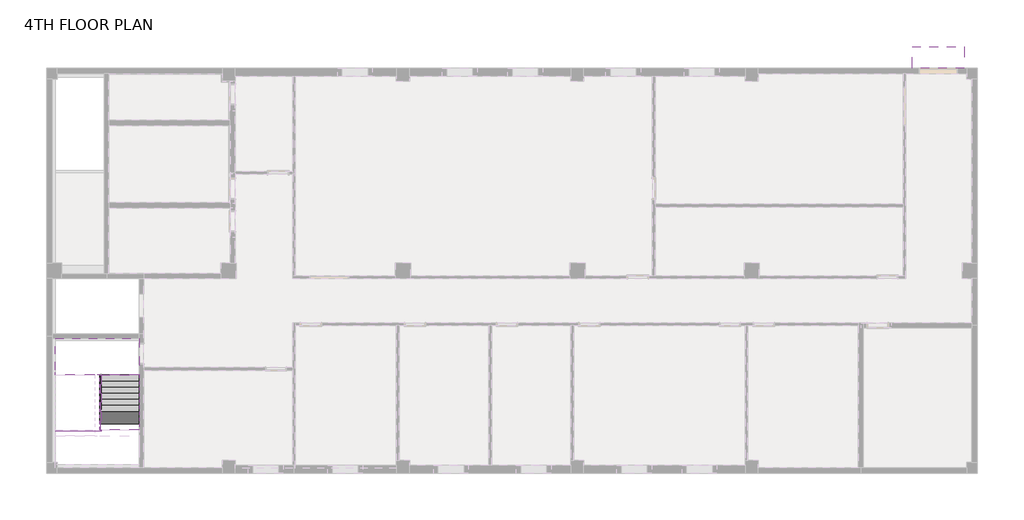
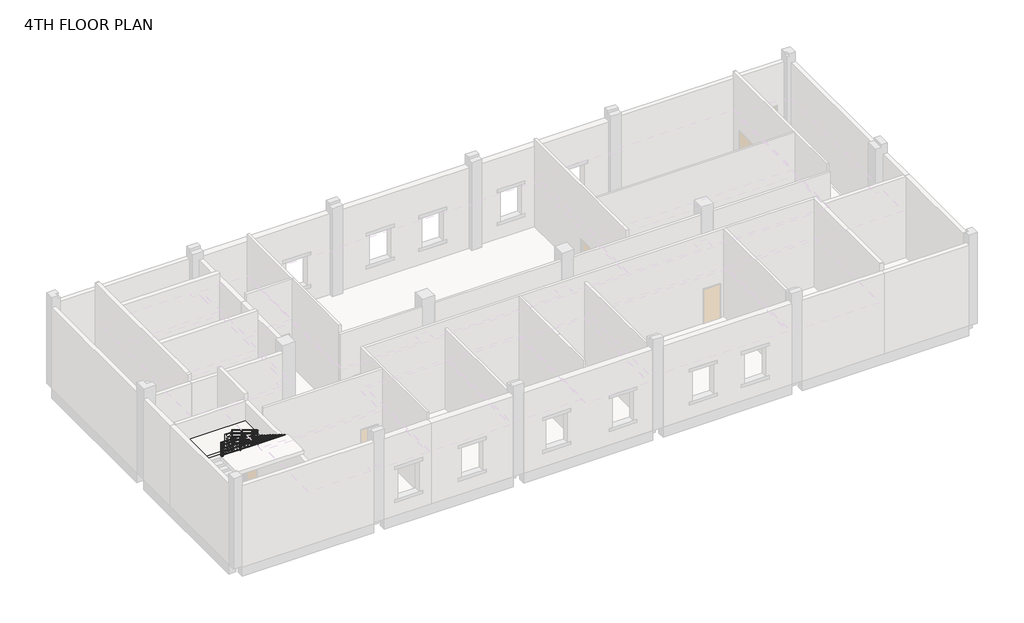
# One storey, part 6 of 6: 2 stair flights, 1 proxy, 1 railing, 1 slab.
"""IFC4 building model written with IfcOpenShell, lengths in millimetres."""

import ifcopenshell
import ifcopenshell.guid

model = None  # the IFC model being written
_history = None  # IfcOwnerHistory: only IFC2X3 demands one
_inside = {}  # id of a spatial element -> (the spatial element, [elements in it])
_under = {}  # id of a project, library or spatial element -> (it, [spatial elements below it])
_declared = {}  # id of a project -> (the project, [libraries it declares])
_typed = {}  # id of a type object -> (the type object, [elements of that type])
_made_of = {}  # id of a material, layer set ... -> (it, [elements and type objects made of it])


def new_model(schema):
    """Start an empty IFC model of exactly this schema.

    Asked for "IFC4X3", IfcOpenShell would pick the latest addendum, in which some entities
    have other attributes; the version numbers below select the first issue.
    IFC2X3 requires an IfcOwnerHistory on every rooted entity: one is made here for all.
    """
    global model, _history
    if schema == "IFC4X3":
        model = ifcopenshell.file(schema_version=(4, 3, 0, 0))
    else:
        model = ifcopenshell.file(schema=schema)
    _inside.clear()
    _under.clear()
    _declared.clear()
    _typed.clear()
    _made_of.clear()
    _history = None
    if model.schema == "IFC2X3":
        org = make("IfcOrganization", Name="unknown")
        user = make(
            "IfcPersonAndOrganization",
            ThePerson=make("IfcPerson", FamilyName="unknown"),
            TheOrganization=org,
        )
        app = make(
            "IfcApplication",
            ApplicationDeveloper=org,
            Version="unknown",
            ApplicationFullName="unknown",
            ApplicationIdentifier="unknown",
        )
        _history = make(
            "IfcOwnerHistory",
            OwningUser=user,
            OwningApplication=app,
            ChangeAction="ADDED",
            CreationDate=0,
        )
    return model


def make(cls, **values):
    """One entity of the class cls with the attributes given. An attribute that is None is left unset."""
    return model.create_entity(
        cls, **{name: value for name, value in values.items() if value is not None}
    )


def rooted(cls, **values):
    """An entity with a GlobalId (a new one), such as an element, a storey or a relation."""
    return make(cls, GlobalId=ifcopenshell.guid.new(), OwnerHistory=_history, **values)


def si_unit(unit_type, name, prefix=None):
    """IfcSIUnit, for example si_unit("LENGTHUNIT", "METRE", prefix="MILLI")."""
    return make("IfcSIUnit", UnitType=unit_type, Prefix=prefix, Name=name)


def assignment(units):
    """IfcUnitAssignment: the units of a project."""
    return None if units is None else make("IfcUnitAssignment", Units=units)


def point(xyz):
    """IfcCartesianPoint."""
    return None if xyz is None else make("IfcCartesianPoint", Coordinates=xyz)


def direction(xyz):
    """IfcDirection."""
    return None if xyz is None else make("IfcDirection", DirectionRatios=xyz)


def frame(location, z_axis=None, x_axis=None):
    """IfcAxis2Placement3D, a coordinate frame: its origin and axes. An axis left out is left unset."""
    return make(
        "IfcAxis2Placement3D",
        Location=point(location),
        Axis=direction(z_axis),
        RefDirection=direction(x_axis),
    )


def origin():
    """The frame at (0, 0, 0) with its axes left unset."""
    return frame((0.0, 0.0, 0.0))


def place(relative_to, where):
    """IfcLocalPlacement: puts the frame where relative to a parent placement (None: the world)."""
    return make(
        "IfcLocalPlacement", PlacementRelTo=relative_to, RelativePlacement=where
    )


def context(
    kind, dimensions, precision=None, world=None, true_north=None, identifier=None
):
    """IfcGeometricRepresentationContext, for example the 3D "Model" context."""
    return make(
        "IfcGeometricRepresentationContext",
        ContextIdentifier=identifier,
        ContextType=kind,
        CoordinateSpaceDimension=dimensions,
        Precision=precision,
        WorldCoordinateSystem=world,
        TrueNorth=true_north,
    )


def project(units=None, contexts=None):
    """IfcProject with its units and contexts."""
    return rooted(
        "IfcProject",
        Name="project",
        RepresentationContexts=contexts,
        UnitsInContext=assignment(units),
    )


def spatial(cls, under=None, at=None, **own):
    """A site, building, storey or space (cls), placed at a placement, below another one or the project."""
    s = rooted(cls, ObjectPlacement=at, **own)
    if under is not None:
        _under.setdefault(under.id(), (under, []))[1].append(s)
    return s


def polyline(points):
    """IfcPolyline through the points."""
    return make("IfcPolyline", Points=[point(p) for p in points])


def circle_curve(where, radius):
    """IfcCircle in the frame where."""
    return make("IfcCircle", Position=where, Radius=radius)


def ellipse_curve(where, semi_axis1, semi_axis2):
    """IfcEllipse in the frame where."""
    return make(
        "IfcEllipse", Position=where, SemiAxis1=semi_axis1, SemiAxis2=semi_axis2
    )


def outline(outer, holes=None, kind="AREA"):
    """IfcArbitraryClosedProfileDef: a profile drawn as a closed curve; with holes, ...WithVoids."""
    if holes is None:
        return make("IfcArbitraryClosedProfileDef", ProfileType=kind, OuterCurve=outer)
    return make(
        "IfcArbitraryProfileDefWithVoids",
        ProfileType=kind,
        OuterCurve=outer,
        InnerCurves=holes,
    )


def extrude(swept, where, along, depth):
    """IfcExtrudedAreaSolid: the profile swept, set in the frame where, extruded along a direction by depth."""
    return make(
        "IfcExtrudedAreaSolid",
        SweptArea=swept,
        Position=where,
        ExtrudedDirection=direction(along),
        Depth=depth,
    )


def faces_of(points, faces, orient=None, outer=None):
    """IfcFace entities. A face is a list of loops; a loop is a list of indices into points, from 0.

    orient and outer hold one flag for each loop. By default every Orientation is true, the
    first loop of a face is its IfcFaceOuterBound and the others are IfcFaceBound.
    """
    made = []
    for i, loops in enumerate(faces):
        bounds = []
        for j, loop in enumerate(loops):
            is_outer = j == 0 if outer is None else outer[i][j]
            bounds.append(
                make(
                    "IfcFaceOuterBound" if is_outer else "IfcFaceBound",
                    Bound=make("IfcPolyLoop", Polygon=[points[k] for k in loop]),
                    Orientation=True if orient is None else orient[i][j],
                )
            )
        made.append(make("IfcFace", Bounds=bounds))
    return made


def faceted_brep(points, faces, orient=None, outer=None, voids=None):
    """IfcFacetedBrep: a solid bounded by flat faces; with voids (closed shells), ...WithVoids."""
    shared = [point(p) for p in points]
    hull = make("IfcClosedShell", CfsFaces=faces_of(shared, faces, orient, outer))
    if voids is None:
        return make("IfcFacetedBrep", Outer=hull)
    return make(
        "IfcFacetedBrepWithVoids",
        Outer=hull,
        Voids=[
            make(cls, CfsFaces=faces_of(shared, fs, o, b)) for cls, fs, o, b in voids
        ],
    )


def shape(context_of_items, identifier, shape_type, items):
    """IfcShapeRepresentation: the items that make up one representation, for example the "Body"."""
    return make(
        "IfcShapeRepresentation",
        ContextOfItems=context_of_items,
        RepresentationIdentifier=identifier,
        RepresentationType=shape_type,
        Items=items,
    )


def source(mapping_origin, context_of_items, identifier, shape_type, items):
    """IfcRepresentationMap: a shape defined once, which mapped items show again and again."""
    return make(
        "IfcRepresentationMap",
        MappingOrigin=mapping_origin,
        MappedRepresentation=shape(context_of_items, identifier, shape_type, items),
    )


def transform(
    local_origin,
    x_axis=None,
    y_axis=None,
    z_axis=None,
    scale=None,
    scale2=None,
    scale3=None,
    uniform=True,
):
    """IfcCartesianTransformationOperator3D, or its non-uniform kind. x_axis, y_axis, z_axis: its Axis1, 2, 3."""
    if uniform:
        return make(
            "IfcCartesianTransformationOperator3D",
            Axis1=direction(x_axis),
            Axis2=direction(y_axis),
            LocalOrigin=point(local_origin),
            Scale=scale,
            Axis3=direction(z_axis),
        )
    return make(
        "IfcCartesianTransformationOperator3DnonUniform",
        Axis1=direction(x_axis),
        Axis2=direction(y_axis),
        LocalOrigin=point(local_origin),
        Scale=scale,
        Axis3=direction(z_axis),
        Scale2=scale2,
        Scale3=scale3,
    )


def mapped(mapping_source, mapping_target):
    """IfcMappedItem: shows the shape of a source again, moved by a transform."""
    return make(
        "IfcMappedItem", MappingSource=mapping_source, MappingTarget=mapping_target
    )


def made_of(thing, what):
    """Note that an element or type object is made of a material, layer set ...; save() writes the relation."""
    if what is not None:
        _made_of.setdefault(what.id(), (what, []))[1].append(thing)
    return thing


def element(
    cls,
    number,
    at=None,
    inside=None,
    cuts=None,
    type_object=None,
    material=None,
    context=None,
    identifier="Body",
    shape_type=None,
    held_by="IfcProductDefinitionShape",
    body=None,
    shapes=None,
    **own,
):
    """One element of the class cls, such as IfcWall. Its Tag is "e" and its number.

    at: its placement. inside: the storey or other place that contains it. cuts: it is an
    opening in that element (IfcRelVoidsElement). A single representation is given by context,
    identifier, shape_type and body (its items); several are given by shapes. held_by: the class
    of the entity that holds the representations. save() writes the other relations.
    """
    e = rooted(cls, Tag="e%d" % number, ObjectPlacement=at, **own)
    if body is not None:
        shapes = [shape(context, identifier, shape_type, body)]
    if shapes is not None:
        e.Representation = make(held_by, Representations=shapes)
    if inside is not None:
        _inside.setdefault(inside.id(), (inside, []))[1].append(e)
    if cuts is not None:
        rooted(
            "IfcRelVoidsElement", RelatingBuildingElement=cuts, RelatedOpeningElement=e
        )
    if type_object is not None:
        _typed.setdefault(type_object.id(), (type_object, []))[1].append(e)
    return made_of(e, material)


def aggregate(whole, parts):
    """IfcRelAggregates: a whole, such as a stair, and the parts it consists of."""
    return rooted("IfcRelAggregates", RelatingObject=whole, RelatedObjects=parts)


def save(model, path):
    """Write the relations noted so far, then the file.

    IfcRelAggregates (storeys below a building ...), IfcRelContainedInSpatialStructure (elements
    in a storey), IfcRelDefinesByType, IfcRelAssociatesMaterial and IfcRelDeclares: one each for
    every whole, place, type object, material and project.
    """
    for whole, parts in _under.values():
        aggregate(whole, parts)
    for where, things in _inside.values():
        rooted(
            "IfcRelContainedInSpatialStructure",
            RelatedElements=things,
            RelatingStructure=where,
        )
    for kind, things in _typed.values():
        rooted("IfcRelDefinesByType", RelatedObjects=things, RelatingType=kind)
    for what, things in _made_of.values():
        rooted("IfcRelAssociatesMaterial", RelatedObjects=things, RelatingMaterial=what)
    for by, libraries in _declared.values():
        rooted("IfcRelDeclares", RelatingContext=by, RelatedDefinitions=libraries)
    model.write(path)


def plane_surface(at):
    """IfcPlane: the flat surface through the origin of the frame at, square to its z axis."""
    return make("IfcPlane", Position=at)


def cylinder_surface(at, radius):
    """IfcCylindricalSurface: all points at the distance radius from the z axis of the frame at."""
    return make("IfcCylindricalSurface", Position=at, Radius=radius)


def advanced_brep(points, edges, surfaces, faces):
    """IfcAdvancedBrep: a solid bounded by faces that lie on surfaces and meet in shared edges.

    An edge is (start, end): straight between two places in points (the first is 0);
    or (start, end, curve); or (start, end, curve, False) where it runs against its curve.
    A face is (place in surfaces, loops), or (place, loops, False) where it looks against
    its surface's normal. A loop lists edges by number (the first is 1), with a minus sign
    where the edge is run from its end to its start. The first loop is the outer one.
    """
    corners = [point(p) for p in points]
    vertices = [make("IfcVertexPoint", VertexGeometry=c) for c in corners]
    made = []
    for start, end, *more in edges:
        made.append(
            make(
                "IfcEdgeCurve",
                EdgeStart=vertices[start],
                EdgeEnd=vertices[end],
                EdgeGeometry=more[0] if more else make("IfcPolyline", Points=[corners[start], corners[end]]),
                SameSense=more[1] if len(more) > 1 else True,
            )
        )
    hull = []
    for where, loops, *sense in faces:
        bounds = []
        for j, loop in enumerate(loops):
            ring = [make("IfcOrientedEdge", EdgeElement=made[abs(k) - 1], Orientation=k > 0) for k in loop]
            bounds.append(
                make(
                    "IfcFaceOuterBound" if j == 0 else "IfcFaceBound",
                    Bound=make("IfcEdgeLoop", EdgeList=ring),
                    Orientation=True,
                )
            )
        hull.append(make("IfcAdvancedFace", Bounds=bounds, FaceSurface=surfaces[where], SameSense=sense[0] if sense else True))
    return make("IfcAdvancedBrep", Outer=make("IfcClosedShell", CfsFaces=hull))


def canopy_no_lintel2_canopy_no_lintel_c6626c79(model_context):
    return source(origin(), model_context, "Body", "SweptSolid", [
        extrude(outline(polyline([(-30.0, 1000.0), (0.0, 0.0), (-150.0, 0.0), (-150.0, 1000.0), (-30.0, 1000.0)])), frame((0.0, 0.0, 0.0), z_axis=(1.0, 0.0, 0.0), x_axis=(0.0, 1.0, 0.0)), (0.0, 0.0, 1.0), 2400.0),
    ])


model = new_model("IFC4")

# Units and contexts
model_context = context("Model", 3, world=origin())
ifc_project = project(units=[si_unit("LENGTHUNIT", "METRE", prefix="MILLI")], contexts=[model_context])

# Site, building, storey
site = spatial("IfcSite", under=ifc_project)
building = spatial("IfcBuilding", under=site)
storey = spatial("IfcBuildingStorey", under=building, Name="4TH FLOOR PLAN", Elevation=16100.005241)

# Proxy
placement = place(None, origin())
canopy_no_lintel2_canopy_no_lintel_shape = canopy_no_lintel2_canopy_no_lintel_c6626c79(model_context)
element("IfcBuildingElementProxy", 1, Name="Canopy_no_ Lintel2 : Canopy No Lintel", ObjectType="Canopy_no_ Lintel2 : Canopy No Lintel", at=placement, inside=storey, context=model_context, shape_type="MappedRepresentation", body=[
    mapped(canopy_no_lintel2_canopy_no_lintel_shape, transform((41750.0, 39300.5208589, 18900.005241), x_axis=(-1.0, 0.0, 0.0), y_axis=(0.0, 0.0, 1.0), z_axis=(0.0, 1.0, 0.0))),
])

# Railing
element("IfcRailing", 2, ObjectType="900mm 배관", at=placement, inside=storey, context=model_context, shape_type="SolidModel", body=[
    advanced_brep(
    [(2135.0, 25213.5208589, 20935.5296813), (2165.0, 25213.5208589, 20935.5296813), (2135.0, 22689.2843108, 22485.005241), (2165.0, 22689.2843108, 22485.005241), (2135.0, 22658.5208589, 22485.005241), (2165.0, 22628.5208589, 22485.005241), (50.0, 22658.5208589, 22485.005241), (50.0, 22628.5208589, 22485.005241)],
    [
        (0, 1, ellipse_curve(frame((2150.0, 25213.5208589, 20935.5296813), z_axis=(0.0, 1.0, 0.0), x_axis=(0.0, 0.0, -1.0)), 17.6005597, 15.0)),
        (1, 0, ellipse_curve(frame((2150.0, 25213.5208589, 20935.5296813), z_axis=(0.0, 1.0, 0.0), x_axis=(0.0, 0.0, -1.0)), 17.6005597, 15.0)),
        (0, 2),
        (2, 3, ellipse_curve(frame((2150.0, 22689.2843108, 22485.005241), z_axis=(0.0, 0.9623527489128064, -0.2718035810285896), x_axis=(0.0, -0.27180358102858976, -0.9623527489128063)), 15.5868002, 15.0)),
        (3, 1),
        (3, 2, ellipse_curve(frame((2150.0, 22689.2843108, 22485.005241), z_axis=(0.0, 0.9623527489128064, -0.2718035810285896), x_axis=(0.0, -0.27180358102858976, -0.9623527489128063)), 15.5868002, 15.0)),
        (2, 4),
        (4, 5, ellipse_curve(frame((2150.0, 22643.5208589, 22485.005241), z_axis=(0.7071067811865475, 0.7071067811865475, 0.0), x_axis=(-0.7071067811865474, 0.7071067811865476, 0.0)), 21.2132034, 15.0)),
        (5, 3),
        (5, 4, ellipse_curve(frame((2150.0, 22643.5208589, 22485.005241), z_axis=(0.7071067811865475, 0.7071067811865475, 0.0), x_axis=(-0.7071067811865474, 0.7071067811865476, 0.0)), 21.2132034, 15.0)),
        (6, 7, circle_curve(frame((50.0, 22643.5208589, 22485.005241), z_axis=(-1.0, 0.0, 0.0), x_axis=(0.0, -1.0, 0.0)), 15.0)),
        (7, 6, circle_curve(frame((50.0, 22643.5208589, 22485.005241), z_axis=(-1.0, 0.0, 0.0), x_axis=(0.0, -1.0, 0.0)), 15.0)),
        (4, 6),
        (7, 5),
    ],
    [
        plane_surface(frame((2150.0, 25213.5208589, 20953.130241), z_axis=(0.0, 1.0, 0.0), x_axis=(0.0, 0.0, -1.0))),
        cylinder_surface(frame((2150.0, 25205.6737312, 20940.3465566), z_axis=(0.0, 0.8522456266800699, -0.5231418467344159), x_axis=(1.0, 0.0, 0.0)), 15.0),
        cylinder_surface(frame((2150.0, 22693.5208589, 22485.005241), z_axis=(0.0, 1.0, 0.0), x_axis=(1.0, 0.0, 0.0)), 15.0),
        plane_surface(frame((50.0, 22643.5208589, 22500.005241), z_axis=(-1.0, 0.0, 0.0), x_axis=(0.0, -1.0, 0.0))),
        cylinder_surface(frame((2150.0, 22643.5208589, 22485.005241), z_axis=(1.0, 0.0, 0.0), x_axis=(0.0, -1.0, 0.0)), 15.0),
    ],
    [
        (0, [[1, 2]]),
        (1, [[-1, 3, 4, 5]]),
        (1, [[-2, -5, 6, -3]]),
        (2, [[-4, 7, 8, 9]]),
        (2, [[-6, -9, 10, -7]]),
        (3, [[11, 12]]),
        (4, [[-8, 13, -12, 14]]),
        (4, [[-10, -14, -11, -13]]),
    ],
),
    advanced_brep(
    [(2165.0, 25213.5208589, 20735.5296813), (2135.0, 25213.5208589, 20735.5296813), (2165.0, 22689.2843108, 22285.005241), (2135.0, 22689.2843108, 22285.005241), (2165.0, 22658.5208589, 22285.005241), (2135.0, 22658.5208589, 22285.005241)],
    [
        (0, 1, ellipse_curve(frame((2150.0, 25213.5208589, 20735.5296813), z_axis=(0.0, 1.0, 0.0), x_axis=(0.0, 0.0, -1.0)), 17.6005597, 15.0)),
        (1, 0, ellipse_curve(frame((2150.0, 25213.5208589, 20735.5296813), z_axis=(0.0, 1.0, 0.0), x_axis=(0.0, 0.0, -1.0)), 17.6005597, 15.0)),
        (0, 2),
        (2, 3, ellipse_curve(frame((2150.0, 22689.2843108, 22285.005241), z_axis=(0.0, 0.9623527489128064, -0.2718035810285896), x_axis=(0.0, -0.27180358102858976, -0.9623527489128063)), 15.5868002, 15.0)),
        (3, 1),
        (3, 2, ellipse_curve(frame((2150.0, 22689.2843108, 22285.005241), z_axis=(0.0, 0.9623527489128064, -0.2718035810285896), x_axis=(0.0, -0.27180358102858976, -0.9623527489128063)), 15.5868002, 15.0)),
        (4, 5, circle_curve(frame((2150.0, 22658.5208589, 22285.005241), z_axis=(0.0, -1.0, 0.0), x_axis=(-1.0, 0.0, 0.0)), 15.0)),
        (5, 4, circle_curve(frame((2150.0, 22658.5208589, 22285.005241), z_axis=(0.0, -1.0, 0.0), x_axis=(-1.0, 0.0, 0.0)), 15.0)),
        (2, 4),
        (5, 3),
    ],
    [
        plane_surface(frame((2150.0, 25213.5208589, 20753.130241), z_axis=(0.0, 1.0, 0.0), x_axis=(0.0, 0.0, -1.0))),
        cylinder_surface(frame((2150.0, 25205.6737312, 20740.3465566), z_axis=(0.0, 0.8522456266800699, -0.5231418467344159), x_axis=(-1.0, 0.0, 0.0)), 15.0),
        plane_surface(frame((2150.0, 22658.5208589, 22300.005241), z_axis=(0.0, -1.0, 0.0), x_axis=(0.0, 0.0, -1.0))),
        cylinder_surface(frame((2150.0, 22693.5208589, 22285.005241), z_axis=(0.0, 1.0, 0.0), x_axis=(-1.0, 0.0, 0.0)), 15.0),
    ],
    [
        (0, [[1, 2]]),
        (1, [[-1, 3, 4, 5]]),
        (1, [[-2, -5, 6, -3]]),
        (2, [[7, 8]]),
        (3, [[-4, 9, -8, 10]]),
        (3, [[-6, -10, -7, -9]]),
    ],
),
    advanced_brep(
    [(2165.0, 25213.5208589, 20535.5296813), (2135.0, 25213.5208589, 20535.5296813), (2165.0, 22689.2843108, 22085.005241), (2135.0, 22689.2843108, 22085.005241), (2165.0, 22658.5208589, 22085.005241), (2135.0, 22658.5208589, 22085.005241)],
    [
        (0, 1, ellipse_curve(frame((2150.0, 25213.5208589, 20535.5296813), z_axis=(0.0, 1.0, 0.0), x_axis=(0.0, 0.0, -1.0)), 17.6005597, 15.0)),
        (1, 0, ellipse_curve(frame((2150.0, 25213.5208589, 20535.5296813), z_axis=(0.0, 1.0, 0.0), x_axis=(0.0, 0.0, -1.0)), 17.6005597, 15.0)),
        (0, 2),
        (2, 3, ellipse_curve(frame((2150.0, 22689.2843108, 22085.005241), z_axis=(0.0, 0.9623527489128064, -0.2718035810285896), x_axis=(0.0, -0.27180358102858976, -0.9623527489128063)), 15.5868002, 15.0)),
        (3, 1),
        (3, 2, ellipse_curve(frame((2150.0, 22689.2843108, 22085.005241), z_axis=(0.0, 0.9623527489128064, -0.2718035810285896), x_axis=(0.0, -0.27180358102858976, -0.9623527489128063)), 15.5868002, 15.0)),
        (4, 5, circle_curve(frame((2150.0, 22658.5208589, 22085.005241), z_axis=(0.0, -1.0, 0.0), x_axis=(-1.0, 0.0, 0.0)), 15.0)),
        (5, 4, circle_curve(frame((2150.0, 22658.5208589, 22085.005241), z_axis=(0.0, -1.0, 0.0), x_axis=(-1.0, 0.0, 0.0)), 15.0)),
        (2, 4),
        (5, 3),
    ],
    [
        plane_surface(frame((2150.0, 25213.5208589, 20553.130241), z_axis=(0.0, 1.0, 0.0), x_axis=(0.0, 0.0, -1.0))),
        cylinder_surface(frame((2150.0, 25205.6737312, 20540.3465566), z_axis=(0.0, 0.8522456266800699, -0.5231418467344159), x_axis=(-1.0, 0.0, 0.0)), 15.0),
        plane_surface(frame((2150.0, 22658.5208589, 22100.005241), z_axis=(0.0, -1.0, 0.0), x_axis=(0.0, 0.0, -1.0))),
        cylinder_surface(frame((2150.0, 22693.5208589, 22085.005241), z_axis=(0.0, 1.0, 0.0), x_axis=(-1.0, 0.0, 0.0)), 15.0),
    ],
    [
        (0, [[1, 2]]),
        (1, [[-1, 3, 4, 5]]),
        (1, [[-2, -5, 6, -3]]),
        (2, [[7, 8]]),
        (3, [[-4, 9, -8, 10]]),
        (3, [[-6, -10, -7, -9]]),
    ],
),
    advanced_brep(
    [(2165.0, 25213.5208589, 20335.5296813), (2135.0, 25213.5208589, 20335.5296813), (2165.0, 22689.2843108, 21885.005241), (2135.0, 22689.2843108, 21885.005241), (2165.0, 22658.5208589, 21885.005241), (2135.0, 22658.5208589, 21885.005241)],
    [
        (0, 1, ellipse_curve(frame((2150.0, 25213.5208589, 20335.5296813), z_axis=(0.0, 1.0, 0.0), x_axis=(0.0, 0.0, -1.0)), 17.6005597, 15.0)),
        (1, 0, ellipse_curve(frame((2150.0, 25213.5208589, 20335.5296813), z_axis=(0.0, 1.0, 0.0), x_axis=(0.0, 0.0, -1.0)), 17.6005597, 15.0)),
        (0, 2),
        (2, 3, ellipse_curve(frame((2150.0, 22689.2843108, 21885.005241), z_axis=(0.0, 0.9623527489128064, -0.2718035810285896), x_axis=(0.0, -0.27180358102858976, -0.9623527489128063)), 15.5868002, 15.0)),
        (3, 1),
        (3, 2, ellipse_curve(frame((2150.0, 22689.2843108, 21885.005241), z_axis=(0.0, 0.9623527489128064, -0.2718035810285896), x_axis=(0.0, -0.27180358102858976, -0.9623527489128063)), 15.5868002, 15.0)),
        (4, 5, circle_curve(frame((2150.0, 22658.5208589, 21885.005241), z_axis=(0.0, -1.0, 0.0), x_axis=(-1.0, 0.0, 0.0)), 15.0)),
        (5, 4, circle_curve(frame((2150.0, 22658.5208589, 21885.005241), z_axis=(0.0, -1.0, 0.0), x_axis=(-1.0, 0.0, 0.0)), 15.0)),
        (2, 4),
        (5, 3),
    ],
    [
        plane_surface(frame((2150.0, 25213.5208589, 20353.130241), z_axis=(0.0, 1.0, 0.0), x_axis=(0.0, 0.0, -1.0))),
        cylinder_surface(frame((2150.0, 25205.6737312, 20340.3465566), z_axis=(0.0, 0.8522456266800699, -0.5231418467344159), x_axis=(-1.0, 0.0, 0.0)), 15.0),
        plane_surface(frame((2150.0, 22658.5208589, 21900.005241), z_axis=(0.0, -1.0, 0.0), x_axis=(0.0, 0.0, -1.0))),
        cylinder_surface(frame((2150.0, 22693.5208589, 21885.005241), z_axis=(0.0, 1.0, 0.0), x_axis=(-1.0, 0.0, 0.0)), 15.0),
    ],
    [
        (0, [[1, 2]]),
        (1, [[-1, 3, 4, 5]]),
        (1, [[-2, -5, 6, -3]]),
        (2, [[7, 8]]),
        (3, [[-4, 9, -8, 10]]),
        (3, [[-6, -10, -7, -9]]),
    ],
),
    advanced_brep(
    [(2165.0, 25213.5208589, 20135.5296813), (2135.0, 25213.5208589, 20135.5296813), (2165.0, 22689.2843108, 21685.005241), (2135.0, 22689.2843108, 21685.005241), (2165.0, 22658.5208589, 21685.005241), (2135.0, 22658.5208589, 21685.005241)],
    [
        (0, 1, ellipse_curve(frame((2150.0, 25213.5208589, 20135.5296813), z_axis=(0.0, 1.0, 0.0), x_axis=(0.0, 0.0, -1.0)), 17.6005597, 15.0)),
        (1, 0, ellipse_curve(frame((2150.0, 25213.5208589, 20135.5296813), z_axis=(0.0, 1.0, 0.0), x_axis=(0.0, 0.0, -1.0)), 17.6005597, 15.0)),
        (0, 2),
        (2, 3, ellipse_curve(frame((2150.0, 22689.2843108, 21685.005241), z_axis=(0.0, 0.9623527489128064, -0.2718035810285896), x_axis=(0.0, -0.27180358102858976, -0.9623527489128063)), 15.5868002, 15.0)),
        (3, 1),
        (3, 2, ellipse_curve(frame((2150.0, 22689.2843108, 21685.005241), z_axis=(0.0, 0.9623527489128064, -0.2718035810285896), x_axis=(0.0, -0.27180358102858976, -0.9623527489128063)), 15.5868002, 15.0)),
        (4, 5, circle_curve(frame((2150.0, 22658.5208589, 21685.005241), z_axis=(0.0, -1.0, 0.0), x_axis=(-1.0, 0.0, 0.0)), 15.0)),
        (5, 4, circle_curve(frame((2150.0, 22658.5208589, 21685.005241), z_axis=(0.0, -1.0, 0.0), x_axis=(-1.0, 0.0, 0.0)), 15.0)),
        (2, 4),
        (5, 3),
    ],
    [
        plane_surface(frame((2150.0, 25213.5208589, 20153.130241), z_axis=(0.0, 1.0, 0.0), x_axis=(0.0, 0.0, -1.0))),
        cylinder_surface(frame((2150.0, 25205.6737312, 20140.3465566), z_axis=(0.0, 0.8522456266800699, -0.5231418467344159), x_axis=(-1.0, 0.0, 0.0)), 15.0),
        plane_surface(frame((2150.0, 22658.5208589, 21700.005241), z_axis=(0.0, -1.0, 0.0), x_axis=(0.0, 0.0, -1.0))),
        cylinder_surface(frame((2150.0, 22693.5208589, 21685.005241), z_axis=(0.0, 1.0, 0.0), x_axis=(-1.0, 0.0, 0.0)), 15.0),
    ],
    [
        (0, [[1, 2]]),
        (1, [[-1, 3, 4, 5]]),
        (1, [[-2, -5, 6, -3]]),
        (2, [[7, 8]]),
        (3, [[-4, 9, -8, 10]]),
        (3, [[-6, -10, -7, -9]]),
    ],
),
    advanced_brep(
    [(2165.0, 22628.5208589, 22285.005241), (2165.0, 22658.5208589, 22285.005241), (50.0, 22628.5208589, 22285.005241), (50.0, 22658.5208589, 22285.005241)],
    [
        (0, 1, circle_curve(frame((2165.0, 22643.5208589, 22285.005241), z_axis=(1.0, 0.0, 0.0), x_axis=(0.0, 1.0, 0.0)), 15.0)),
        (1, 0, circle_curve(frame((2165.0, 22643.5208589, 22285.005241), z_axis=(1.0, 0.0, 0.0), x_axis=(0.0, 1.0, 0.0)), 15.0)),
        (2, 3, circle_curve(frame((50.0, 22643.5208589, 22285.005241), z_axis=(-1.0, 0.0, 0.0), x_axis=(0.0, 1.0, 0.0)), 15.0)),
        (3, 2, circle_curve(frame((50.0, 22643.5208589, 22285.005241), z_axis=(-1.0, 0.0, 0.0), x_axis=(0.0, 1.0, 0.0)), 15.0)),
        (0, 2),
        (3, 1),
    ],
    [
        plane_surface(frame((2165.0, 22643.5208589, 22300.005241), z_axis=(1.0, 0.0, 0.0), x_axis=(0.0, -1.0, 0.0))),
        plane_surface(frame((50.0, 22643.5208589, 22300.005241), z_axis=(-1.0, 0.0, 0.0), x_axis=(0.0, -1.0, 0.0))),
        cylinder_surface(frame((2165.0, 22643.5208589, 22285.005241), z_axis=(1.0, 0.0, 0.0), x_axis=(0.0, 1.0, 0.0)), 15.0),
    ],
    [
        (0, [[1, 2]]),
        (1, [[3, 4]]),
        (2, [[-1, 5, -4, 6]]),
        (2, [[-2, -6, -3, -5]]),
    ],
),
    advanced_brep(
    [(2165.0, 22628.5208589, 22085.005241), (2165.0, 22658.5208589, 22085.005241), (50.0, 22628.5208589, 22085.005241), (50.0, 22658.5208589, 22085.005241)],
    [
        (0, 1, circle_curve(frame((2165.0, 22643.5208589, 22085.005241), z_axis=(1.0, 0.0, 0.0), x_axis=(0.0, 1.0, 0.0)), 15.0)),
        (1, 0, circle_curve(frame((2165.0, 22643.5208589, 22085.005241), z_axis=(1.0, 0.0, 0.0), x_axis=(0.0, 1.0, 0.0)), 15.0)),
        (2, 3, circle_curve(frame((50.0, 22643.5208589, 22085.005241), z_axis=(-1.0, 0.0, 0.0), x_axis=(0.0, 1.0, 0.0)), 15.0)),
        (3, 2, circle_curve(frame((50.0, 22643.5208589, 22085.005241), z_axis=(-1.0, 0.0, 0.0), x_axis=(0.0, 1.0, 0.0)), 15.0)),
        (0, 2),
        (3, 1),
    ],
    [
        plane_surface(frame((2165.0, 22643.5208589, 22100.005241), z_axis=(1.0, 0.0, 0.0), x_axis=(0.0, -1.0, 0.0))),
        plane_surface(frame((50.0, 22643.5208589, 22100.005241), z_axis=(-1.0, 0.0, 0.0), x_axis=(0.0, -1.0, 0.0))),
        cylinder_surface(frame((2165.0, 22643.5208589, 22085.005241), z_axis=(1.0, 0.0, 0.0), x_axis=(0.0, 1.0, 0.0)), 15.0),
    ],
    [
        (0, [[1, 2]]),
        (1, [[3, 4]]),
        (2, [[-1, 5, -4, 6]]),
        (2, [[-2, -6, -3, -5]]),
    ],
),
    advanced_brep(
    [(2165.0, 22628.5208589, 21885.005241), (2165.0, 22658.5208589, 21885.005241), (50.0, 22628.5208589, 21885.005241), (50.0, 22658.5208589, 21885.005241)],
    [
        (0, 1, circle_curve(frame((2165.0, 22643.5208589, 21885.005241), z_axis=(1.0, 0.0, 0.0), x_axis=(0.0, 1.0, 0.0)), 15.0)),
        (1, 0, circle_curve(frame((2165.0, 22643.5208589, 21885.005241), z_axis=(1.0, 0.0, 0.0), x_axis=(0.0, 1.0, 0.0)), 15.0)),
        (2, 3, circle_curve(frame((50.0, 22643.5208589, 21885.005241), z_axis=(-1.0, 0.0, 0.0), x_axis=(0.0, 1.0, 0.0)), 15.0)),
        (3, 2, circle_curve(frame((50.0, 22643.5208589, 21885.005241), z_axis=(-1.0, 0.0, 0.0), x_axis=(0.0, 1.0, 0.0)), 15.0)),
        (0, 2),
        (3, 1),
    ],
    [
        plane_surface(frame((2165.0, 22643.5208589, 21900.005241), z_axis=(1.0, 0.0, 0.0), x_axis=(0.0, -1.0, 0.0))),
        plane_surface(frame((50.0, 22643.5208589, 21900.005241), z_axis=(-1.0, 0.0, 0.0), x_axis=(0.0, -1.0, 0.0))),
        cylinder_surface(frame((2165.0, 22643.5208589, 21885.005241), z_axis=(1.0, 0.0, 0.0), x_axis=(0.0, 1.0, 0.0)), 15.0),
    ],
    [
        (0, [[1, 2]]),
        (1, [[3, 4]]),
        (2, [[-1, 5, -4, 6]]),
        (2, [[-2, -6, -3, -5]]),
    ],
),
    advanced_brep(
    [(2165.0, 22628.5208589, 21685.005241), (2165.0, 22658.5208589, 21685.005241), (50.0, 22628.5208589, 21685.005241), (50.0, 22658.5208589, 21685.005241)],
    [
        (0, 1, circle_curve(frame((2165.0, 22643.5208589, 21685.005241), z_axis=(1.0, 0.0, 0.0), x_axis=(0.0, 1.0, 0.0)), 15.0)),
        (1, 0, circle_curve(frame((2165.0, 22643.5208589, 21685.005241), z_axis=(1.0, 0.0, 0.0), x_axis=(0.0, 1.0, 0.0)), 15.0)),
        (2, 3, circle_curve(frame((50.0, 22643.5208589, 21685.005241), z_axis=(-1.0, 0.0, 0.0), x_axis=(0.0, 1.0, 0.0)), 15.0)),
        (3, 2, circle_curve(frame((50.0, 22643.5208589, 21685.005241), z_axis=(-1.0, 0.0, 0.0), x_axis=(0.0, 1.0, 0.0)), 15.0)),
        (0, 2),
        (3, 1),
    ],
    [
        plane_surface(frame((2165.0, 22643.5208589, 21700.005241), z_axis=(1.0, 0.0, 0.0), x_axis=(0.0, -1.0, 0.0))),
        plane_surface(frame((50.0, 22643.5208589, 21700.005241), z_axis=(-1.0, 0.0, 0.0), x_axis=(0.0, -1.0, 0.0))),
        cylinder_surface(frame((2165.0, 22643.5208589, 21685.005241), z_axis=(1.0, 0.0, 0.0), x_axis=(0.0, 1.0, 0.0)), 15.0),
    ],
    [
        (0, [[1, 2]]),
        (1, [[3, 4]]),
        (2, [[-1, 5, -4, 6]]),
        (2, [[-2, -6, -3, -5]]),
    ],
),
    extrude(outline(polyline([(162.5, 22656.0208589), (162.5, 22631.0208589), (137.5, 22631.0208589), (137.5, 22656.0208589), (162.5, 22656.0208589)])), frame((0.0, 0.0, 21600.005241), z_axis=(0.0, 0.0, 1.0), x_axis=(1.0, 0.0, 0.0)), (0.0, 0.0, 1.0), 870.0),
    extrude(outline(polyline([(1162.5, 22656.0208589), (1162.5, 22631.0208589), (1137.5, 22631.0208589), (1137.5, 22656.0208589), (1162.5, 22656.0208589)])), frame((0.0, 0.0, 21600.005241), z_axis=(0.0, 0.0, 1.0), x_axis=(1.0, 0.0, 0.0)), (0.0, 0.0, 1.0), 870.0),
    extrude(outline(polyline([(23201.0208589, 22153.2806841), (23226.0208589, 22137.934702), (23226.0208589, 21256.255241), (23201.0208589, 21256.255241), (23201.0208589, 22153.2806841)])), frame((2137.5, 0.0, 0.0), z_axis=(1.0, 0.0, 0.0), x_axis=(0.0, 1.0, 0.0)), (0.0, 0.0, 1.0), 25.0),
    extrude(outline(polyline([(24201.0208589, 21539.4413984), (24226.0208589, 21524.0954163), (24226.0208589, 20568.755241), (24201.0208589, 20568.755241), (24201.0208589, 21539.4413984)])), frame((2137.5, 0.0, 0.0), z_axis=(1.0, 0.0, 0.0), x_axis=(0.0, 1.0, 0.0)), (0.0, 0.0, 1.0), 25.0),
    extrude(outline(polyline([(2137.5, 22656.0208589), (2162.5, 22656.0208589), (2162.5, 22631.0208589), (2137.5, 22631.0208589), (2137.5, 22656.0208589)])), frame((0.0, 0.0, 21600.005241), z_axis=(0.0, 0.0, 1.0), x_axis=(1.0, 0.0, 0.0)), (0.0, 0.0, 1.0), 870.0),
    extrude(outline(polyline([(75.0, 22656.0208589), (75.0, 22631.0208589), (50.0, 22631.0208589), (50.0, 22656.0208589), (75.0, 22656.0208589)])), frame((0.0, 0.0, 21600.005241), z_axis=(0.0, 0.0, 1.0), x_axis=(1.0, 0.0, 0.0)), (0.0, 0.0, 1.0), 870.0),
    extrude(outline(polyline([(25188.5208589, 20933.2751038), (25213.5208589, 20917.9291216), (25213.5208589, 20053.130241), (25188.5208589, 20053.130241), (25188.5208589, 20933.2751038)])), frame((2137.5, 0.0, 0.0), z_axis=(1.0, 0.0, 0.0), x_axis=(0.0, 1.0, 0.0)), (0.0, 0.0, 1.0), 25.0),
])

# Slab
element("IfcSlab", 3, ObjectType="프리캐스트 콘크리트 - 200mm 두께", at=placement, inside=storey, context=model_context, shape_type="SolidModel", body=[
    faceted_brep([(50.0, 25213.5208589, 19880.461491), (1850.0, 25213.5208589, 19880.461491), (2100.0, 25213.5208589, 19880.461491), (3900.0, 25213.5208589, 19880.461491), (3900.0, 25252.6099233, 19880.461491), (3900.0, 26899.5208589, 19880.461491), (50.0, 26899.5208589, 19880.461491), (50.0, 25454.4317945, 19880.461491), (50.0, 25213.5208589, 19708.586491), (50.0, 25213.5208589, 19532.5808943), (1850.0, 25213.5208589, 19532.5808943), (1850.0, 25213.5208589, 19680.461491), (2100.0, 25213.5208589, 19680.461491), (2100.0, 25213.5208589, 19704.4558943), (3900.0, 25213.5208589, 19704.4558943), (3900.0, 25252.6099233, 19680.461491), (3900.0, 26899.5208589, 19680.461491), (50.0, 26899.5208589, 19680.461491), (50.0, 25454.4317945, 19680.461491), (2100.0, 25252.6099233, 19680.461491), (1850.0, 25454.4317945, 19680.461491)], [[[0, 1, 2, 3, 4, 5, 6, 7]], [[1, 0, 8, 9, 10, 11]], [[2, 1, 11, 12, 13]], [[3, 14, 15, 16, 5, 4]], [[6, 5, 16, 17]], [[9, 8, 0, 7, 6, 17, 18]], [[19, 12, 11, 20, 18, 17, 16, 15]], [[12, 19, 13]], [[18, 20, 10, 9]], [[20, 11, 10]], [[19, 15, 14, 13]], [[3, 2, 13, 14]]]),
    extrude(outline(polyline([(50.0, 25213.5208589), (50.0, 26899.5208589), (3900.0, 26899.5208589), (3900.0, 25213.5208589), (2100.0, 25213.5208589), (1850.0, 25213.5208589), (50.0, 25213.5208589)])), frame((0.0, 0.0, 19880.461491), z_axis=(0.0, 0.0, 1.0), x_axis=(1.0, 0.0, 0.0)), (0.0, 0.0, 1.0), 0.79375),
])

# Stair flights
element("IfcStairFlight", 4, ObjectType="1mm 디딤판", at=placement, inside=storey, context=model_context, shape_type="SolidModel", body=[
    faceted_brep([(3900.0, 24933.5208589, 16271.086491), (3900.0, 25213.5208589, 16271.086491), (2100.0, 25213.5208589, 16271.086491), (2100.0, 24933.5208589, 16271.086491), (3900.0, 24933.5208589, 16100.005241), (3900.0, 25213.5208589, 16100.005241), (2100.0, 25213.5208589, 16100.005241), (2100.0, 24933.5208589, 16100.005241), (3900.0, 24653.5208589, 16442.961491), (3900.0, 24933.5208589, 16442.961491), (2100.0, 24933.5208589, 16442.961491), (2100.0, 24653.5208589, 16442.961491), (3900.0, 24653.5208589, 16266.9558943), (3900.0, 24925.4986506, 16100.005241), (2100.0, 24925.4986506, 16100.005241), (2100.0, 24653.5208589, 16266.9558943), (3900.0, 24373.5208589, 16614.836491), (3900.0, 24653.5208589, 16614.836491), (2100.0, 24653.5208589, 16614.836491), (2100.0, 24373.5208589, 16614.836491), (3900.0, 24373.5208589, 16438.8308943), (2100.0, 24373.5208589, 16438.8308943), (3900.0, 24093.5208589, 16786.711491), (3900.0, 24373.5208589, 16786.711491), (2100.0, 24373.5208589, 16786.711491), (2100.0, 24093.5208589, 16786.711491), (3900.0, 24093.5208589, 16610.7058943), (2100.0, 24093.5208589, 16610.7058943), (3900.0, 23813.5208589, 16958.586491), (3900.0, 24093.5208589, 16958.586491), (2100.0, 24093.5208589, 16958.586491), (2100.0, 23813.5208589, 16958.586491), (3900.0, 23813.5208589, 16782.5808943), (2100.0, 23813.5208589, 16782.5808943), (3900.0, 23533.5208589, 17130.461491), (3900.0, 23813.5208589, 17130.461491), (2100.0, 23813.5208589, 17130.461491), (2100.0, 23533.5208589, 17130.461491), (3900.0, 23533.5208589, 16954.4558943), (2100.0, 23533.5208589, 16954.4558943), (3900.0, 23253.5208589, 17302.336491), (3900.0, 23533.5208589, 17302.336491), (2100.0, 23533.5208589, 17302.336491), (2100.0, 23253.5208589, 17302.336491), (3900.0, 23253.5208589, 17126.3308943), (2100.0, 23253.5208589, 17126.3308943), (3900.0, 22973.5208589, 17474.211491), (3900.0, 23253.5208589, 17474.211491), (2100.0, 23253.5208589, 17474.211491), (2100.0, 22973.5208589, 17474.211491), (3900.0, 22973.5208589, 17298.2058943), (2100.0, 22973.5208589, 17298.2058943), (3900.0, 22693.5208589, 17646.086491), (3900.0, 22973.5208589, 17646.086491), (2100.0, 22973.5208589, 17646.086491), (2100.0, 22693.5208589, 17646.086491), (3900.0, 22693.5208589, 17470.0808943), (2100.0, 22693.5208589, 17470.0808943), (3900.0, 22413.5208589, 17817.961491), (3900.0, 22693.5208589, 17817.961491), (2100.0, 22693.5208589, 17817.961491), (2100.0, 22413.5208589, 17817.961491), (3900.0, 22413.5208589, 17641.9558943), (2100.0, 22413.5208589, 17641.9558943), (2100.0, 22413.5208589, 17789.836491)], [[[0, 1, 2, 3]], [[1, 0, 4, 5]], [[2, 1, 5, 6]], [[3, 2, 6, 7]], [[8, 9, 10, 11]], [[4, 0, 9, 8, 12, 13]], [[0, 3, 10, 9]], [[3, 7, 14, 15, 11, 10]], [[16, 17, 18, 19]], [[17, 16, 20, 12, 8]], [[8, 11, 18, 17]], [[19, 18, 11, 15, 21]], [[22, 23, 24, 25]], [[23, 22, 26, 20, 16]], [[16, 19, 24, 23]], [[25, 24, 19, 21, 27]], [[28, 29, 30, 31]], [[29, 28, 32, 26, 22]], [[22, 25, 30, 29]], [[31, 30, 25, 27, 33]], [[34, 35, 36, 37]], [[35, 34, 38, 32, 28]], [[28, 31, 36, 35]], [[37, 36, 31, 33, 39]], [[40, 41, 42, 43]], [[41, 40, 44, 38, 34]], [[34, 37, 42, 41]], [[43, 42, 37, 39, 45]], [[46, 47, 48, 49]], [[47, 46, 50, 44, 40]], [[40, 43, 48, 47]], [[49, 48, 43, 45, 51]], [[52, 53, 54, 55]], [[53, 52, 56, 50, 46]], [[46, 49, 54, 53]], [[55, 54, 49, 51, 57]], [[58, 59, 60, 61]], [[59, 58, 62, 56, 52]], [[52, 55, 60, 59]], [[61, 60, 55, 57, 63, 64]], [[58, 61, 64, 63, 62]], [[5, 4, 13, 14, 7, 6]], [[14, 13, 12, 20, 26, 32, 38, 44, 50, 56, 62, 63, 57, 51, 45, 39, 33, 27, 21, 15]]]),
    extrude(outline(polyline([(3900.0, 24933.5208589), (2100.0, 24933.5208589), (2100.0, 25213.5208589), (3900.0, 25213.5208589), (3900.0, 24933.5208589)])), frame((0.0, 0.0, 16271.086491), z_axis=(0.0, 0.0, 1.0), x_axis=(1.0, 0.0, 0.0)), (0.0, 0.0, 1.0), 0.79375),
    extrude(outline(polyline([(3900.0, 24653.5208589), (2100.0, 24653.5208589), (2100.0, 24933.5208589), (3900.0, 24933.5208589), (3900.0, 24653.5208589)])), frame((0.0, 0.0, 16442.961491), z_axis=(0.0, 0.0, 1.0), x_axis=(1.0, 0.0, 0.0)), (0.0, 0.0, 1.0), 0.79375),
    extrude(outline(polyline([(3900.0, 24373.5208589), (2100.0, 24373.5208589), (2100.0, 24653.5208589), (3900.0, 24653.5208589), (3900.0, 24373.5208589)])), frame((0.0, 0.0, 16614.836491), z_axis=(0.0, 0.0, 1.0), x_axis=(1.0, 0.0, 0.0)), (0.0, 0.0, 1.0), 0.79375),
    extrude(outline(polyline([(3900.0, 24093.5208589), (2100.0, 24093.5208589), (2100.0, 24373.5208589), (3900.0, 24373.5208589), (3900.0, 24093.5208589)])), frame((0.0, 0.0, 16786.711491), z_axis=(0.0, 0.0, 1.0), x_axis=(1.0, 0.0, 0.0)), (0.0, 0.0, 1.0), 0.79375),
    extrude(outline(polyline([(3900.0, 23813.5208589), (2100.0, 23813.5208589), (2100.0, 24093.5208589), (3900.0, 24093.5208589), (3900.0, 23813.5208589)])), frame((0.0, 0.0, 16958.586491), z_axis=(0.0, 0.0, 1.0), x_axis=(1.0, 0.0, 0.0)), (0.0, 0.0, 1.0), 0.79375),
    extrude(outline(polyline([(3900.0, 23533.5208589), (2100.0, 23533.5208589), (2100.0, 23813.5208589), (3900.0, 23813.5208589), (3900.0, 23533.5208589)])), frame((0.0, 0.0, 17130.461491), z_axis=(0.0, 0.0, 1.0), x_axis=(1.0, 0.0, 0.0)), (0.0, 0.0, 1.0), 0.79375),
    extrude(outline(polyline([(3900.0, 23253.5208589), (2100.0, 23253.5208589), (2100.0, 23533.5208589), (3900.0, 23533.5208589), (3900.0, 23253.5208589)])), frame((0.0, 0.0, 17302.336491), z_axis=(0.0, 0.0, 1.0), x_axis=(1.0, 0.0, 0.0)), (0.0, 0.0, 1.0), 0.79375),
    extrude(outline(polyline([(3900.0, 22973.5208589), (2100.0, 22973.5208589), (2100.0, 23253.5208589), (3900.0, 23253.5208589), (3900.0, 22973.5208589)])), frame((0.0, 0.0, 17474.211491), z_axis=(0.0, 0.0, 1.0), x_axis=(1.0, 0.0, 0.0)), (0.0, 0.0, 1.0), 0.79375),
    extrude(outline(polyline([(3900.0, 22693.5208589), (2100.0, 22693.5208589), (2100.0, 22973.5208589), (3900.0, 22973.5208589), (3900.0, 22693.5208589)])), frame((0.0, 0.0, 17646.086491), z_axis=(0.0, 0.0, 1.0), x_axis=(1.0, 0.0, 0.0)), (0.0, 0.0, 1.0), 0.79375),
    extrude(outline(polyline([(3900.0, 22413.5208589), (2100.0, 22413.5208589), (2100.0, 22693.5208589), (3900.0, 22693.5208589), (3900.0, 22413.5208589)])), frame((0.0, 0.0, 17817.961491), z_axis=(0.0, 0.0, 1.0), x_axis=(1.0, 0.0, 0.0)), (0.0, 0.0, 1.0), 0.79375),
])
element("IfcStairFlight", 5, ObjectType="1mm 디딤판", at=placement, inside=storey, context=model_context, shape_type="SolidModel", body=[
    faceted_brep([(3900.0, 24933.5208589, 20052.336491), (3900.0, 25213.5208589, 20052.336491), (2100.0, 25213.5208589, 20052.336491), (2100.0, 24933.5208589, 20052.336491), (3900.0, 24933.5208589, 19876.3308943), (3900.0, 25213.5208589, 19704.4558943), (3900.0, 25213.5208589, 19880.461491), (2100.0, 25213.5208589, 19704.4558943), (2100.0, 24933.5208589, 19876.3308943), (3900.0, 24653.5208589, 20224.211491), (3900.0, 24933.5208589, 20224.211491), (2100.0, 24933.5208589, 20224.211491), (2100.0, 24653.5208589, 20224.211491), (3900.0, 24653.5208589, 20048.2058943), (2100.0, 24653.5208589, 20048.2058943), (3900.0, 24373.5208589, 20396.086491), (3900.0, 24653.5208589, 20396.086491), (2100.0, 24653.5208589, 20396.086491), (2100.0, 24373.5208589, 20396.086491), (3900.0, 24373.5208589, 20220.0808943), (2100.0, 24373.5208589, 20220.0808943), (3900.0, 24093.5208589, 20567.961491), (3900.0, 24373.5208589, 20567.961491), (2100.0, 24373.5208589, 20567.961491), (2100.0, 24093.5208589, 20567.961491), (3900.0, 24093.5208589, 20391.9558943), (2100.0, 24093.5208589, 20391.9558943), (3900.0, 23813.5208589, 20739.836491), (3900.0, 24093.5208589, 20739.836491), (2100.0, 24093.5208589, 20739.836491), (2100.0, 23813.5208589, 20739.836491), (3900.0, 23813.5208589, 20563.8308943), (2100.0, 23813.5208589, 20563.8308943), (3900.0, 23533.5208589, 20911.711491), (3900.0, 23813.5208589, 20911.711491), (2100.0, 23813.5208589, 20911.711491), (2100.0, 23533.5208589, 20911.711491), (3900.0, 23533.5208589, 20735.7058943), (2100.0, 23533.5208589, 20735.7058943), (3900.0, 23253.5208589, 21083.586491), (3900.0, 23533.5208589, 21083.586491), (2100.0, 23533.5208589, 21083.586491), (2100.0, 23253.5208589, 21083.586491), (3900.0, 23253.5208589, 20907.5808943), (2100.0, 23253.5208589, 20907.5808943), (3900.0, 22973.5208589, 21255.461491), (3900.0, 23253.5208589, 21255.461491), (2100.0, 23253.5208589, 21255.461491), (2100.0, 22973.5208589, 21255.461491), (3900.0, 22973.5208589, 21079.4558943), (2100.0, 22973.5208589, 21079.4558943), (3900.0, 22693.5208589, 21427.336491), (3900.0, 22973.5208589, 21427.336491), (2100.0, 22973.5208589, 21427.336491), (2100.0, 22693.5208589, 21427.336491), (3900.0, 22693.5208589, 21251.3308943), (2100.0, 22693.5208589, 21251.3308943), (2100.0, 22693.5208589, 21399.211491)], [[[0, 1, 2, 3]], [[1, 0, 4, 5, 6]], [[2, 1, 6, 5, 7]], [[3, 2, 7, 8]], [[9, 10, 11, 12]], [[10, 9, 13, 4, 0]], [[11, 10, 0, 3]], [[12, 11, 3, 8, 14]], [[15, 16, 17, 18]], [[16, 15, 19, 13, 9]], [[17, 16, 9, 12]], [[18, 17, 12, 14, 20]], [[21, 22, 23, 24]], [[22, 21, 25, 19, 15]], [[23, 22, 15, 18]], [[24, 23, 18, 20, 26]], [[27, 28, 29, 30]], [[28, 27, 31, 25, 21]], [[29, 28, 21, 24]], [[30, 29, 24, 26, 32]], [[33, 34, 35, 36]], [[34, 33, 37, 31, 27]], [[35, 34, 27, 30]], [[36, 35, 30, 32, 38]], [[39, 40, 41, 42]], [[40, 39, 43, 37, 33]], [[41, 40, 33, 36]], [[42, 41, 36, 38, 44]], [[45, 46, 47, 48]], [[46, 45, 49, 43, 39]], [[47, 46, 39, 42]], [[48, 47, 42, 44, 50]], [[51, 52, 53, 54]], [[52, 51, 55, 49, 45]], [[53, 52, 45, 48]], [[54, 53, 48, 50, 56, 57]], [[51, 54, 57, 56, 55]], [[5, 4, 13, 19, 25, 31, 37, 43, 49, 55, 56, 50, 44, 38, 32, 26, 20, 14, 8, 7]]]),
    extrude(outline(polyline([(3900.0, 24933.5208589), (2100.0, 24933.5208589), (2100.0, 25213.5208589), (3900.0, 25213.5208589), (3900.0, 24933.5208589)])), frame((0.0, 0.0, 20052.336491), z_axis=(0.0, 0.0, 1.0), x_axis=(1.0, 0.0, 0.0)), (0.0, 0.0, 1.0), 0.79375),
    extrude(outline(polyline([(3900.0, 24653.5208589), (2100.0, 24653.5208589), (2100.0, 24933.5208589), (3900.0, 24933.5208589), (3900.0, 24653.5208589)])), frame((0.0, 0.0, 20224.211491), z_axis=(0.0, 0.0, 1.0), x_axis=(1.0, 0.0, 0.0)), (0.0, 0.0, 1.0), 0.79375),
    extrude(outline(polyline([(3900.0, 24373.5208589), (2100.0, 24373.5208589), (2100.0, 24653.5208589), (3900.0, 24653.5208589), (3900.0, 24373.5208589)])), frame((0.0, 0.0, 20396.086491), z_axis=(0.0, 0.0, 1.0), x_axis=(1.0, 0.0, 0.0)), (0.0, 0.0, 1.0), 0.79375),
    extrude(outline(polyline([(3900.0, 24093.5208589), (2100.0, 24093.5208589), (2100.0, 24373.5208589), (3900.0, 24373.5208589), (3900.0, 24093.5208589)])), frame((0.0, 0.0, 20567.961491), z_axis=(0.0, 0.0, 1.0), x_axis=(1.0, 0.0, 0.0)), (0.0, 0.0, 1.0), 0.79375),
    extrude(outline(polyline([(3900.0, 23813.5208589), (2100.0, 23813.5208589), (2100.0, 24093.5208589), (3900.0, 24093.5208589), (3900.0, 23813.5208589)])), frame((0.0, 0.0, 20739.836491), z_axis=(0.0, 0.0, 1.0), x_axis=(1.0, 0.0, 0.0)), (0.0, 0.0, 1.0), 0.79375),
    extrude(outline(polyline([(3900.0, 23533.5208589), (2100.0, 23533.5208589), (2100.0, 23813.5208589), (3900.0, 23813.5208589), (3900.0, 23533.5208589)])), frame((0.0, 0.0, 20911.711491), z_axis=(0.0, 0.0, 1.0), x_axis=(1.0, 0.0, 0.0)), (0.0, 0.0, 1.0), 0.79375),
    extrude(outline(polyline([(3900.0, 23253.5208589), (2100.0, 23253.5208589), (2100.0, 23533.5208589), (3900.0, 23533.5208589), (3900.0, 23253.5208589)])), frame((0.0, 0.0, 21083.586491), z_axis=(0.0, 0.0, 1.0), x_axis=(1.0, 0.0, 0.0)), (0.0, 0.0, 1.0), 0.79375),
    extrude(outline(polyline([(3900.0, 22973.5208589), (2100.0, 22973.5208589), (2100.0, 23253.5208589), (3900.0, 23253.5208589), (3900.0, 22973.5208589)])), frame((0.0, 0.0, 21255.461491), z_axis=(0.0, 0.0, 1.0), x_axis=(1.0, 0.0, 0.0)), (0.0, 0.0, 1.0), 0.79375),
    extrude(outline(polyline([(3900.0, 22693.5208589), (2100.0, 22693.5208589), (2100.0, 22973.5208589), (3900.0, 22973.5208589), (3900.0, 22693.5208589)])), frame((0.0, 0.0, 21427.336491), z_axis=(0.0, 0.0, 1.0), x_axis=(1.0, 0.0, 0.0)), (0.0, 0.0, 1.0), 0.79375),
])

save(model, "model.ifc")

# Revit data of these elements
# Type "Canopy_no_ Lintel2 : Canopy No Lintel"
#   LastUpdate = "2017-07-05 오후 5:00:05"
#   EditorName = ""
#   lintel width = 413 mm
#   lintel edge = 0 mm
#   lintel depth = 400 mm
#   d2 = 150 mm
#   d1 = 30 mm
#   W = 1000 mm
#   Length [instance default] = 2000 mm
#   Default Elevation = 1219.2 mm
#   Structure Material = none
# Type "900mm 배관"
#   built-in parameter 1008612 = 0.019685 (stored number, unit not read)
#   built-in parameter 1008611 = 0.0984252 (stored number, unit not read)
#   built-in parameter 1008609 = 3.28084 (stored number, unit not read)
#   built-in parameter 1008604 = 0.19685 (stored number, unit not read)
#   built-in parameter 1008603 = 0.164042 (stored number, unit not read)
#   Railing Height = 900 mm
#   built-in parameter 1008630 = 2
#   built-in parameter 1008610 = 1
#   built-in parameter 1008605 = 1
#   built-in parameter 1008618 = 난간동자 - 정사각형1 : 25mm
# Element 1 (IfcBuildingElementProxy, "Canopy_no_ Lintel2 : Canopy No Lintel")
#   Length = 2400 mm
#   Phase Created = New Construction
# Element 2 (IfcRailing, "900mm 배관")
#   Phase Created = New Construction
#   Materials on its faces: "Metal - Stainless Steel,Polished"
# Element 3 (IfcSlab, "프리캐스트 콘크리트 - 200mm 두께")
#   Phase Created = New Construction
#   Materials on its faces: "A03AD032-00007_Structural Concrete_25MPa-30MPa"
# Elements 4, 5 (IfcStairFlight, "1mm 디딤판")
#   Phase Created = New Construction
#   Materials on its faces: "A03AD032-00007_Structural Concrete_25MPa-30MPa"
# Materials
#   "Metal - Stainless Steel,Polished": class "Metal", colour RGB 189 187 185, transparency 0, Description = "STEEL HANDRAIL(TYP.)", Cost = 0
#   "A03AD032-00007_Structural Concrete_25MPa-30MPa": class "Concrete", colour RGB 176 176 176, transparency 0, Keynote = "09910.A1", Description = "ACRYLIC EMULSION PAINT ON\nFAIR FACED CONC.", W00) Work Master Code = "A03AD032-00007", W01) Work Master_Lv1 = "Concrete Work", W02) Work Master_Lv2 = "Superstructure Work", W03) Work Master_Spec.1 = "Structural Concrete", W04) Work Master_Spec.2 = "Cement Type-1", W05) Work Master_Spec.3 = "25MPa < F'c (Cylinder Strength) ≤ 30MPa", Cost = 0
